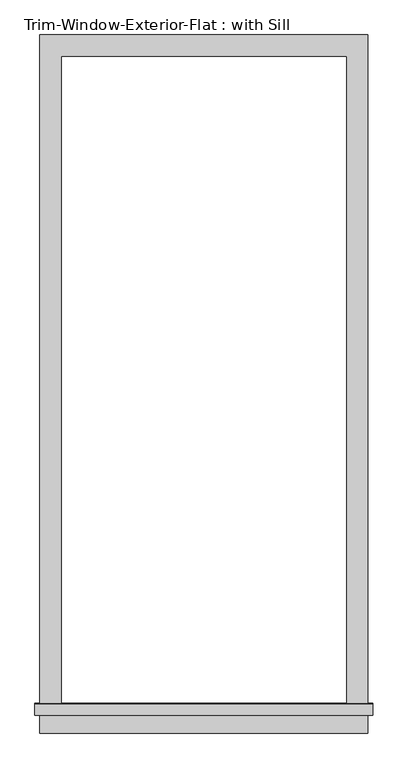
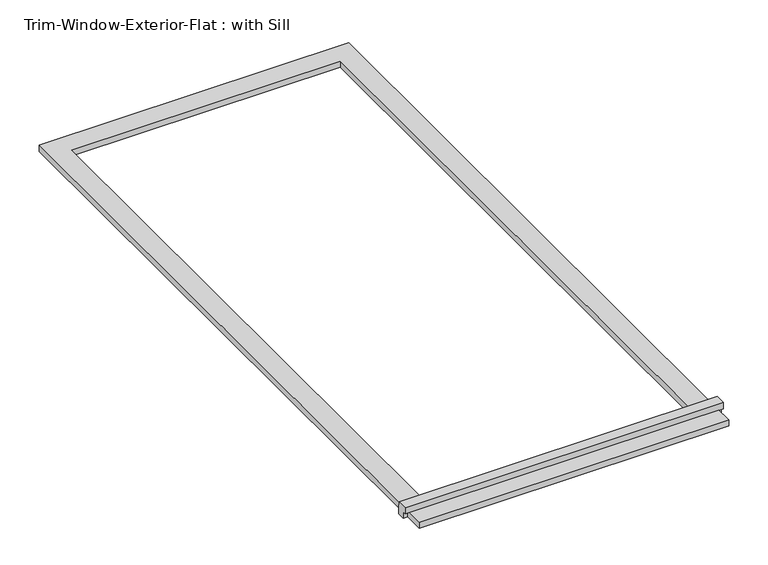
"""IFC4 building model written with IfcOpenShell, lengths in millimetres: proxy geometry, Trim-Window-Exterior-Flat : with Sill."""

import ifcopenshell
import ifcopenshell.guid

model = None  # the IFC model being written
_history = None  # IfcOwnerHistory: only IFC2X3 demands one
_inside = {}  # id of a spatial element -> (the spatial element, [elements in it])
_under = {}  # id of a project, library or spatial element -> (it, [spatial elements below it])
_declared = {}  # id of a project -> (the project, [libraries it declares])
_typed = {}  # id of a type object -> (the type object, [elements of that type])
_made_of = {}  # id of a material, layer set ... -> (it, [elements and type objects made of it])


def new_model(schema):
    """Start an empty IFC model of exactly this schema.

    Asked for "IFC4X3", IfcOpenShell would pick the latest addendum, in which some entities
    have other attributes; the version numbers below select the first issue.
    IFC2X3 requires an IfcOwnerHistory on every rooted entity: one is made here for all.
    """
    global model, _history
    if schema == "IFC4X3":
        model = ifcopenshell.file(schema_version=(4, 3, 0, 0))
    else:
        model = ifcopenshell.file(schema=schema)
    _inside.clear()
    _under.clear()
    _declared.clear()
    _typed.clear()
    _made_of.clear()
    _history = None
    if model.schema == "IFC2X3":
        org = make("IfcOrganization", Name="unknown")
        user = make(
            "IfcPersonAndOrganization",
            ThePerson=make("IfcPerson", FamilyName="unknown"),
            TheOrganization=org,
        )
        app = make(
            "IfcApplication",
            ApplicationDeveloper=org,
            Version="unknown",
            ApplicationFullName="unknown",
            ApplicationIdentifier="unknown",
        )
        _history = make(
            "IfcOwnerHistory",
            OwningUser=user,
            OwningApplication=app,
            ChangeAction="ADDED",
            CreationDate=0,
        )
    return model


def make(cls, **values):
    """One entity of the class cls with the attributes given. An attribute that is None is left unset."""
    return model.create_entity(
        cls, **{name: value for name, value in values.items() if value is not None}
    )


def rooted(cls, **values):
    """An entity with a GlobalId (a new one), such as an element, a storey or a relation."""
    return make(cls, GlobalId=ifcopenshell.guid.new(), OwnerHistory=_history, **values)


def si_unit(unit_type, name, prefix=None):
    """IfcSIUnit, for example si_unit("LENGTHUNIT", "METRE", prefix="MILLI")."""
    return make("IfcSIUnit", UnitType=unit_type, Prefix=prefix, Name=name)


def assignment(units):
    """IfcUnitAssignment: the units of a project."""
    return None if units is None else make("IfcUnitAssignment", Units=units)


def point(xyz):
    """IfcCartesianPoint."""
    return None if xyz is None else make("IfcCartesianPoint", Coordinates=xyz)


def direction(xyz):
    """IfcDirection."""
    return None if xyz is None else make("IfcDirection", DirectionRatios=xyz)


def frame(location, z_axis=None, x_axis=None):
    """IfcAxis2Placement3D, a coordinate frame: its origin and axes. An axis left out is left unset."""
    return make(
        "IfcAxis2Placement3D",
        Location=point(location),
        Axis=direction(z_axis),
        RefDirection=direction(x_axis),
    )


def origin():
    """The frame at (0, 0, 0) with its axes left unset."""
    return frame((0.0, 0.0, 0.0))


def origin_with_axes():
    """The frame at (0, 0, 0) with the z axis (0, 0, 1) and the x axis (1, 0, 0) written out."""
    return frame((0.0, 0.0, 0.0), z_axis=(0.0, 0.0, 1.0), x_axis=(1.0, 0.0, 0.0))


def place(relative_to, where):
    """IfcLocalPlacement: puts the frame where relative to a parent placement (None: the world)."""
    return make(
        "IfcLocalPlacement", PlacementRelTo=relative_to, RelativePlacement=where
    )


def context(
    kind, dimensions, precision=None, world=None, true_north=None, identifier=None
):
    """IfcGeometricRepresentationContext, for example the 3D "Model" context."""
    return make(
        "IfcGeometricRepresentationContext",
        ContextIdentifier=identifier,
        ContextType=kind,
        CoordinateSpaceDimension=dimensions,
        Precision=precision,
        WorldCoordinateSystem=world,
        TrueNorth=true_north,
    )


def project(units=None, contexts=None):
    """IfcProject with its units and contexts."""
    return rooted(
        "IfcProject",
        Name="project",
        RepresentationContexts=contexts,
        UnitsInContext=assignment(units),
    )


def spatial(cls, under=None, at=None, **own):
    """A site, building, storey or space (cls), placed at a placement, below another one or the project."""
    s = rooted(cls, ObjectPlacement=at, **own)
    if under is not None:
        _under.setdefault(under.id(), (under, []))[1].append(s)
    return s


def polyline(points):
    """IfcPolyline through the points."""
    return make("IfcPolyline", Points=[point(p) for p in points])


def outline(outer, holes=None, kind="AREA"):
    """IfcArbitraryClosedProfileDef: a profile drawn as a closed curve; with holes, ...WithVoids."""
    if holes is None:
        return make("IfcArbitraryClosedProfileDef", ProfileType=kind, OuterCurve=outer)
    return make(
        "IfcArbitraryProfileDefWithVoids",
        ProfileType=kind,
        OuterCurve=outer,
        InnerCurves=holes,
    )


def extrude(swept, where, along, depth):
    """IfcExtrudedAreaSolid: the profile swept, set in the frame where, extruded along a direction by depth."""
    return make(
        "IfcExtrudedAreaSolid",
        SweptArea=swept,
        Position=where,
        ExtrudedDirection=direction(along),
        Depth=depth,
    )


def shape(context_of_items, identifier, shape_type, items):
    """IfcShapeRepresentation: the items that make up one representation, for example the "Body"."""
    return make(
        "IfcShapeRepresentation",
        ContextOfItems=context_of_items,
        RepresentationIdentifier=identifier,
        RepresentationType=shape_type,
        Items=items,
    )


def source(mapping_origin, context_of_items, identifier, shape_type, items):
    """IfcRepresentationMap: a shape defined once, which mapped items show again and again."""
    return make(
        "IfcRepresentationMap",
        MappingOrigin=mapping_origin,
        MappedRepresentation=shape(context_of_items, identifier, shape_type, items),
    )


def transform(
    local_origin,
    x_axis=None,
    y_axis=None,
    z_axis=None,
    scale=None,
    scale2=None,
    scale3=None,
    uniform=True,
):
    """IfcCartesianTransformationOperator3D, or its non-uniform kind. x_axis, y_axis, z_axis: its Axis1, 2, 3."""
    if uniform:
        return make(
            "IfcCartesianTransformationOperator3D",
            Axis1=direction(x_axis),
            Axis2=direction(y_axis),
            LocalOrigin=point(local_origin),
            Scale=scale,
            Axis3=direction(z_axis),
        )
    return make(
        "IfcCartesianTransformationOperator3DnonUniform",
        Axis1=direction(x_axis),
        Axis2=direction(y_axis),
        LocalOrigin=point(local_origin),
        Scale=scale,
        Axis3=direction(z_axis),
        Scale2=scale2,
        Scale3=scale3,
    )


def mapped(mapping_source, mapping_target):
    """IfcMappedItem: shows the shape of a source again, moved by a transform."""
    return make(
        "IfcMappedItem", MappingSource=mapping_source, MappingTarget=mapping_target
    )


def made_of(thing, what):
    """Note that an element or type object is made of a material, layer set ...; save() writes the relation."""
    if what is not None:
        _made_of.setdefault(what.id(), (what, []))[1].append(thing)
    return thing


def element(
    cls,
    number,
    at=None,
    inside=None,
    cuts=None,
    type_object=None,
    material=None,
    context=None,
    identifier="Body",
    shape_type=None,
    held_by="IfcProductDefinitionShape",
    body=None,
    shapes=None,
    **own,
):
    """One element of the class cls, such as IfcWall. Its Tag is "e" and its number.

    at: its placement. inside: the storey or other place that contains it. cuts: it is an
    opening in that element (IfcRelVoidsElement). A single representation is given by context,
    identifier, shape_type and body (its items); several are given by shapes. held_by: the class
    of the entity that holds the representations. save() writes the other relations.
    """
    e = rooted(cls, Tag="e%d" % number, ObjectPlacement=at, **own)
    if body is not None:
        shapes = [shape(context, identifier, shape_type, body)]
    if shapes is not None:
        e.Representation = make(held_by, Representations=shapes)
    if inside is not None:
        _inside.setdefault(inside.id(), (inside, []))[1].append(e)
    if cuts is not None:
        rooted(
            "IfcRelVoidsElement", RelatingBuildingElement=cuts, RelatedOpeningElement=e
        )
    if type_object is not None:
        _typed.setdefault(type_object.id(), (type_object, []))[1].append(e)
    return made_of(e, material)


def aggregate(whole, parts):
    """IfcRelAggregates: a whole, such as a stair, and the parts it consists of."""
    return rooted("IfcRelAggregates", RelatingObject=whole, RelatedObjects=parts)


def save(model, path):
    """Write the relations noted so far, then the file.

    IfcRelAggregates (storeys below a building ...), IfcRelContainedInSpatialStructure (elements
    in a storey), IfcRelDefinesByType, IfcRelAssociatesMaterial and IfcRelDeclares: one each for
    every whole, place, type object, material and project.
    """
    for whole, parts in _under.values():
        aggregate(whole, parts)
    for where, things in _inside.values():
        rooted(
            "IfcRelContainedInSpatialStructure",
            RelatedElements=things,
            RelatingStructure=where,
        )
    for kind, things in _typed.values():
        rooted("IfcRelDefinesByType", RelatedObjects=things, RelatingType=kind)
    for what, things in _made_of.values():
        rooted("IfcRelAssociatesMaterial", RelatedObjects=things, RelatingMaterial=what)
    for by, libraries in _declared.values():
        rooted("IfcRelDeclares", RelatingContext=by, RelatedDefinitions=libraries)
    model.write(path)


def trim_window_exterior_flat_with_sill_b28819c4(model_context):
    return source(origin(), model_context, "Body", "SweptSolid", [
        extrude(outline(polyline([(438.15, -1749.3823709), (438.15, -1806.5323709), (-438.15, -1806.5323709), (-438.15, -1749.3823709), (438.15, -1749.3823709)])), origin_with_axes(), (0.0, 0.0, 1.0), 19.05),
        extrude(outline(polyline([(-1758.95, 38.1), (-1729.6580645, 38.1), (-1727.2, 19.05), (-1727.2, 0.0), (-1749.3823709, 0.0), (-1749.3823709, 19.05), (-1758.95, 19.05), (-1758.95, 38.1)])), frame((-450.85, 0.0, 0.0), z_axis=(1.0, 0.0, 0.0), x_axis=(0.0, 1.0, 0.0)), (0.0, 0.0, 1.0), 901.7),
        extrude(outline(polyline([(-438.15, 57.15), (438.15, 57.15), (438.15, -1727.2), (381.0, -1727.2), (381.0, 0.0), (-381.0, 0.0), (-381.0, -1727.2), (-438.15, -1727.2), (-438.15, 57.15)])), origin_with_axes(), (0.0, 0.0, 1.0), 19.05),
    ])


if __name__ == "__main__":
    model = new_model("IFC4")
    model_context = context("Model", 3, world=origin())
    ifc_project = project(units=[si_unit("LENGTHUNIT", "METRE", prefix="MILLI")], contexts=[model_context])
    site = spatial("IfcSite", under=ifc_project)
    building = spatial("IfcBuilding", under=site)
    placement = place(None, origin())
    trim_window_exterior_flat_with_sill_shape = trim_window_exterior_flat_with_sill_b28819c4(model_context)
    element("IfcBuildingElementProxy", 1, Name="Trim-Window-Exterior-Flat : with Sill", ObjectType="Trim-Window-Exterior-Flat : with Sill", at=placement, inside=building, context=model_context, shape_type="MappedRepresentation", body=[
        mapped(trim_window_exterior_flat_with_sill_shape, transform((0.0, 0.0, 0.0), x_axis=(1.0, 0.0, 0.0), y_axis=(0.0, 1.0, 0.0), z_axis=(0.0, 0.0, 1.0))),
    ])
    save(model, "model.ifc")

# Revit data of these elements
# Type "Trim-Window-Exterior-Flat : with Sill"
#   Trim Width = 0' - 2 1/4"
#   Trim Thickness_Picture Frame = 0' - 1 1/4"
#   Trim Thickness_with Sill = 0' - 0 3/4"
#   Sill Thickness = 0' - 1 1/4"
#   Opening Width [instance default] = 2' - 0"
#   Opening Height [instance default] = 3' - 0"
#   Default Elevation = 4' - 0"
#   Sill = yes
#   Picture Frame = no
#   Trim Material [instance default] = none
# Element 1 (IfcBuildingElementProxy, "Trim-Window-Exterior-Flat : with Sill")
#   Opening Width = 2' - 6"
#   Opening Height = 5' - 8"
#   Trim Material = Clad - White
#   Materials on its faces: "Clad - White"
# Materials
#   "Clad - White": class "Wood", colour RGB 242 242 238, transparency 0, Cost = 0
